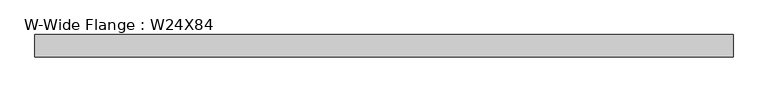
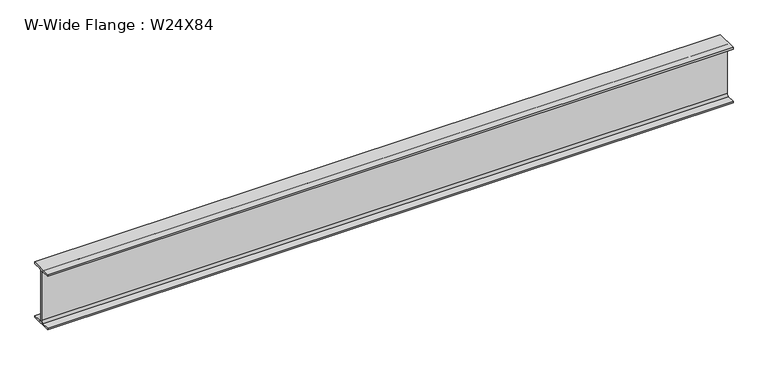
"""IFC4 building model written with IfcOpenShell, lengths in millimetres: beam geometry, W-Wide Flange : W24X84."""

from ifc_helpers import new_model, si_unit, point, frame, frame_2d, origin, place, context, project, spatial, polyline, circle_curve, trimmed, segment, composite_curve, outline, extrude, source, transform, mapped, element, save


def w_wide_flange_w24x84_e470d529(model_context):
    return source(origin(), model_context, "Body", "SweptSolid", [
        extrude(outline(composite_curve([segment(polyline([(114.554, -286.512), (114.554, -306.07), (-114.554, -306.07), (-114.554, -286.512), (-29.2735, -286.512)]), True, "CONTINUOUS"), segment(trimmed(circle_curve(frame_2d((-29.2735, -263.2075)), 23.3045), [point((-29.2735, -286.512))], [point((-5.969, -263.2075))], True, "CARTESIAN"), True, "CONTINUOUS"), segment(polyline([(-5.969, -263.2075), (-5.969, 263.2075)]), True, "CONTINUOUS"), segment(trimmed(circle_curve(frame_2d((-29.2735, 263.2075)), 23.3045), [point((-5.969, 263.2075))], [point((-29.2735, 286.512))], True, "CARTESIAN"), True, "CONTINUOUS"), segment(polyline([(-29.2735, 286.512), (-114.554, 286.512), (-114.554, 306.07), (114.554, 306.07), (114.554, 286.512), (29.2735, 286.512)]), True, "CONTINUOUS"), segment(trimmed(circle_curve(frame_2d((29.2735, 263.2075)), 23.3045), [point((29.2735, 286.512))], [point((5.969, 263.2075))], True, "CARTESIAN"), True, "CONTINUOUS"), segment(polyline([(5.969, 263.2075), (5.969, -263.2075)]), True, "CONTINUOUS"), segment(trimmed(circle_curve(frame_2d((29.2735, -263.2075)), 23.3045), [point((5.969, -263.2075))], [point((29.2735, -286.512))], True, "CARTESIAN"), True, "CONTINUOUS"), segment(polyline([(29.2735, -286.512), (114.554, -286.512)]), True, "CONTINUOUS")], self_intersect=False)), frame((-3510.7066406, 0.0, 0.0), z_axis=(1.0, 0.0, 0.0), x_axis=(0.0, 1.0, 0.0)), (0.0, 0.0, 1.0), 7156.3507813),
    ])


if __name__ == "__main__":
    model = new_model("IFC4")
    model_context = context("Model", 3, world=origin())
    ifc_project = project(units=[si_unit("LENGTHUNIT", "METRE", prefix="MILLI")], contexts=[model_context])
    site = spatial("IfcSite", under=ifc_project)
    building = spatial("IfcBuilding", under=site)
    placement = place(None, origin())
    w_wide_flange_w24x84_shape = w_wide_flange_w24x84_e470d529(model_context)
    element("IfcBeam", 1, ObjectType="W-Wide Flange : W24X84", at=placement, inside=building, context=model_context, shape_type="MappedRepresentation", body=[
        mapped(w_wide_flange_w24x84_shape, transform((0.0, 0.0, 0.0), x_axis=(1.0, 0.0, 0.0), y_axis=(0.0, 1.0, 0.0), z_axis=(0.0, 0.0, 1.0))),
    ])
    save(model, "model.ifc")

# Revit data of these elements
# Type "W-Wide Flange : W24X84"
#   Assembly Code = "B10"
#   W = 84
#   Length [instance default] = 1524 mm
#   bf = 229.108 mm
#   d = 612.14 mm
#   k = 42.863 mm
#   k2 = 23.305 mm
#   tf = 19.558 mm
#   tw = 11.938 mm
#   A = 0.0159355 m²
#   Structural Material [instance default] = Steel ASTM A992
# Element 1 (IfcBeam, "W-Wide Flange : W24X84")
#   Structural Material = Aluminum, Anodized Red
#   Materials on its faces: "Aluminum, Anodized Red"
# Materials
#   "Steel ASTM A992": class "Metal", colour RGB 128 0 0, transparency 0, Description = "Structural steel 50ksi", Cost = 0
#   "Aluminum, Anodized Red": class "Metal", colour RGB 120 120 120, transparency 0, Description = "Anodized aluminum, red", Cost = 0
